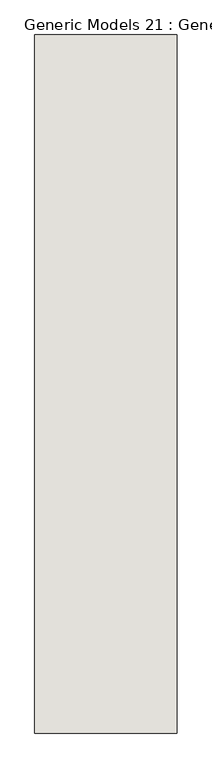
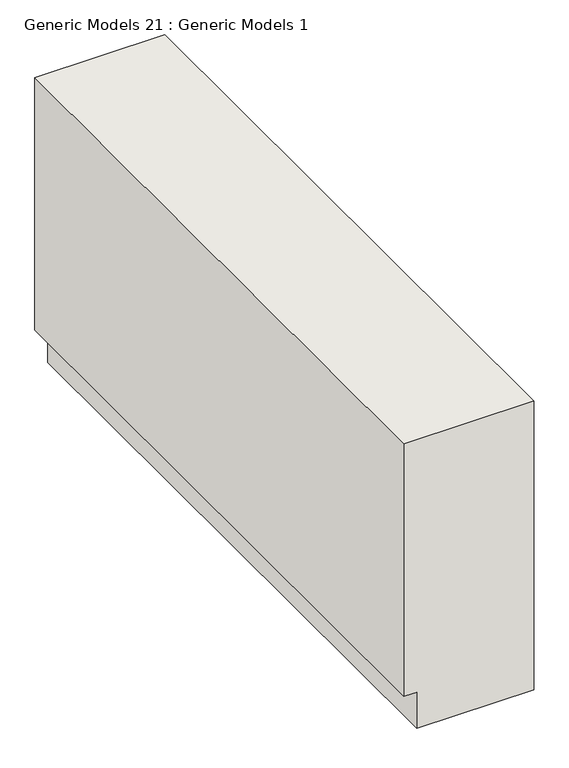
"""IFC4 building model written with IfcOpenShell, lengths in millimetres: wall geometry, Generic Models 21 : Generic Models 1."""

from ifc_helpers import new_model, si_unit, frame, origin, place, context, project, spatial, polyline, outline, extrude, source, transform, mapped, element, save


def generic_models_21_generic_models_1_dc3d701e(model_context):
    return source(origin(), model_context, "Body", "SweptSolid", [
        extrude(outline(polyline([(2452.7089811, 138456.5014063), (3035.6238843, 138456.5014063), (3035.6238843, 138208.1931254), (2525.961714, 138208.1931254), (2525.961714, 138232.7941211), (2452.7089811, 138232.7941211), (2452.7089811, 138456.5014063)])), frame((0.0, 0.0, 0.0), z_axis=(0.0, 1.0, 0.0), x_axis=(0.0, 0.0, 1.0)), (0.0, 0.0, 1.0), 1219.2),
    ])


if __name__ == "__main__":
    model = new_model("IFC4")
    model_context = context("Model", 3, world=origin())
    ifc_project = project(units=[si_unit("LENGTHUNIT", "METRE", prefix="MILLI")], contexts=[model_context])
    site = spatial("IfcSite", under=ifc_project)
    building = spatial("IfcBuilding", under=site)
    placement = place(None, origin())
    generic_models_21_generic_models_1_shape = generic_models_21_generic_models_1_dc3d701e(model_context)
    element("IfcWall", 1, ObjectType="Generic Models 21 : Generic Models 1", at=placement, inside=building, context=model_context, shape_type="MappedRepresentation", body=[
        mapped(generic_models_21_generic_models_1_shape, transform((0.0, 0.0, 0.0), x_axis=(1.0, 0.0, 0.0), y_axis=(0.0, 1.0, 0.0), z_axis=(0.0, 0.0, 1.0))),
    ])
    save(model, "model.ifc")

# Revit data of these elements
# Element 1 (IfcWall, "Generic Models 21 : Generic Models 1")
#   Materials on its faces: "WOOD TRUSS FLOOR ASSEMBLY - FILL CAVITY WITH BATT. INSULATION - (UL - L521 FLOOR ASSEMBLY)"
# Materials
#   "WOOD TRUSS FLOOR ASSEMBLY - FILL CAVITY WITH BATT. INSULATION - (UL - L521 FLOOR ASSEMBLY)": class "Generic", colour RGB 227 188 136, transparency 0, Cost = 0
